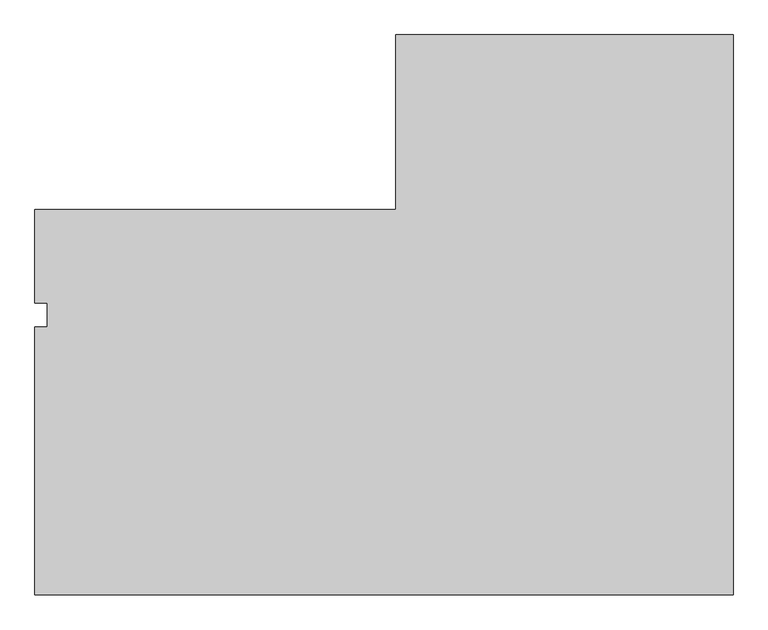
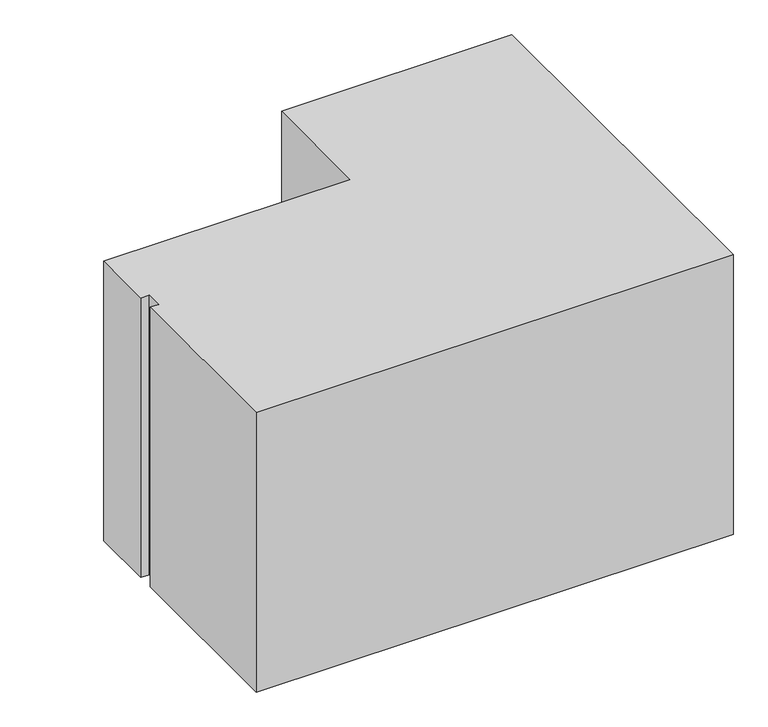
"""IFC4 building model written with IfcOpenShell, lengths in millimetres: proxy geometry, 0_3d."""

from ifc_helpers import new_model, si_unit, origin, origin_with_axes, place, context, project, spatial, polyline, outline, extrude, source, transform, mapped, element, save


def generic_models_b37590e8(model_context):
    return source(origin(), model_context, "Body", "SweptSolid", [
        extrude(outline(polyline([(0.0, 2564.9), (2399.6864914, 2564.9), (2399.6864914, 3726.6), (4642.0, 3726.6), (4642.0, 0.0), (0.0, 0.0), (0.0, 1783.3), (82.0, 1783.3), (82.0, 1943.3), (0.0, 1943.3), (0.0, 2564.9)])), origin_with_axes(), (0.0, 0.0, 1.0), 2880.0),
    ])


if __name__ == "__main__":
    model = new_model("IFC4")
    model_context = context("Model", 3, world=origin())
    ifc_project = project(units=[si_unit("LENGTHUNIT", "METRE", prefix="MILLI")], contexts=[model_context])
    site = spatial("IfcSite", under=ifc_project)
    building = spatial("IfcBuilding", under=site)
    placement = place(None, origin())
    generic_models_shape = generic_models_b37590e8(model_context)
    element("IfcBuildingElementProxy", 1, Name="0_3d", ObjectType="0_3d", at=placement, inside=building, context=model_context, shape_type="MappedRepresentation", body=[
        mapped(generic_models_shape, transform((0.0, 0.0, 0.0), x_axis=(1.0, 0.0, 0.0), y_axis=(0.0, 1.0, 0.0), z_axis=(0.0, 0.0, 1.0))),
    ])
    save(model, "model.ifc")

# Revit data of these elements
# Element 1 (IfcBuildingElementProxy, "0_3d")
#   Materials on its faces: "*1"
# Materials
#   "*1": class "Unassigned", colour RGB 175 175 175, transparency 0
